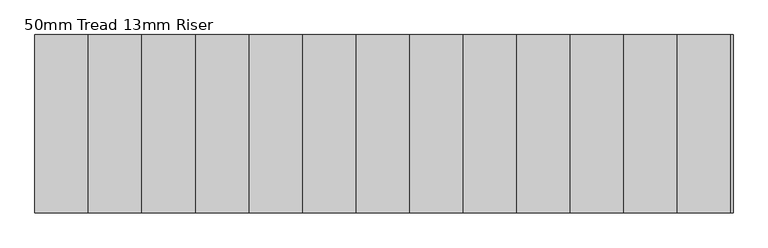
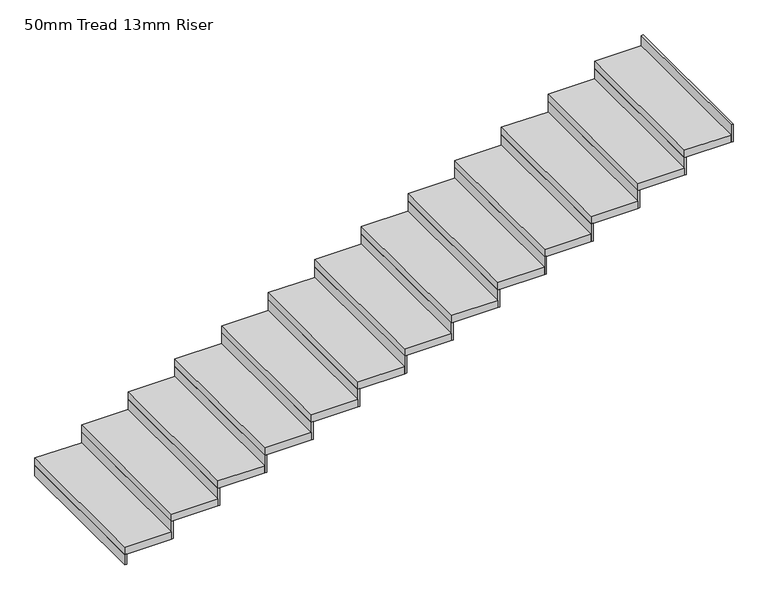
"""IFC4 building model written with IfcOpenShell, lengths in millimetres: stair flight geometry, 50mm Tread 13mm Riser."""

from ifc_helpers import new_model, si_unit, frame, origin, place, context, project, spatial, polyline, outline, extrude, source, transform, mapped, element, save


def stair_flight_50mm_tread_13mm_riser_be5964fb(model_context):
    return source(origin(), model_context, "Body", "SweptSolid", [
        extrude(outline(polyline([(17862.336337, -4574.4857187), (17849.836337, -4574.4857187), (17849.836337, -3574.4857187), (17862.336337, -3574.4857187), (17862.336337, -4574.4857187)])), frame((0.0, 0.0, 3000.0), z_axis=(0.0, 0.0, 1.0), x_axis=(1.0, 0.0, 0.0)), (0.0, 0.0, 1.0), 70.0),
        extrude(outline(polyline([(18149.836337, -3574.4857187), (18149.836337, -4574.4857187), (17849.836337, -4574.4857187), (17849.836337, -3574.4857187), (18149.836337, -3574.4857187)])), frame((0.0, 0.0, 3070.0), z_axis=(0.0, 0.0, 1.0), x_axis=(1.0, 0.0, 0.0)), (0.0, 0.0, 1.0), 50.0),
        extrude(outline(polyline([(18162.336337, -4574.4857187), (18149.836337, -4574.4857187), (18149.836337, -3574.4857187), (18162.336337, -3574.4857187), (18162.336337, -4574.4857187)])), frame((0.0, 0.0, 3070.0), z_axis=(0.0, 0.0, 1.0), x_axis=(1.0, 0.0, 0.0)), (0.0, 0.0, 1.0), 120.0),
        extrude(outline(polyline([(18449.836337, -3574.4857187), (18449.836337, -4574.4857187), (18149.836337, -4574.4857187), (18149.836337, -3574.4857187), (18449.836337, -3574.4857187)])), frame((0.0, 0.0, 3190.0), z_axis=(0.0, 0.0, 1.0), x_axis=(1.0, 0.0, 0.0)), (0.0, 0.0, 1.0), 50.0),
        extrude(outline(polyline([(18462.336337, -4574.4857187), (18449.836337, -4574.4857187), (18449.836337, -3574.4857187), (18462.336337, -3574.4857187), (18462.336337, -4574.4857187)])), frame((0.0, 0.0, 3190.0), z_axis=(0.0, 0.0, 1.0), x_axis=(1.0, 0.0, 0.0)), (0.0, 0.0, 1.0), 120.0),
        extrude(outline(polyline([(18749.836337, -3574.4857187), (18749.836337, -4574.4857187), (18449.836337, -4574.4857187), (18449.836337, -3574.4857187), (18749.836337, -3574.4857187)])), frame((0.0, 0.0, 3310.0), z_axis=(0.0, 0.0, 1.0), x_axis=(1.0, 0.0, 0.0)), (0.0, 0.0, 1.0), 50.0),
        extrude(outline(polyline([(18762.336337, -4574.4857187), (18749.836337, -4574.4857187), (18749.836337, -3574.4857187), (18762.336337, -3574.4857187), (18762.336337, -4574.4857187)])), frame((0.0, 0.0, 3310.0), z_axis=(0.0, 0.0, 1.0), x_axis=(1.0, 0.0, 0.0)), (0.0, 0.0, 1.0), 120.0),
        extrude(outline(polyline([(19049.836337, -3574.4857187), (19049.836337, -4574.4857187), (18749.836337, -4574.4857187), (18749.836337, -3574.4857187), (19049.836337, -3574.4857187)])), frame((0.0, 0.0, 3430.0), z_axis=(0.0, 0.0, 1.0), x_axis=(1.0, 0.0, 0.0)), (0.0, 0.0, 1.0), 50.0),
        extrude(outline(polyline([(19062.336337, -4574.4857187), (19049.836337, -4574.4857187), (19049.836337, -3574.4857187), (19062.336337, -3574.4857187), (19062.336337, -4574.4857187)])), frame((0.0, 0.0, 3430.0), z_axis=(0.0, 0.0, 1.0), x_axis=(1.0, 0.0, 0.0)), (0.0, 0.0, 1.0), 120.0),
        extrude(outline(polyline([(19349.836337, -3574.4857187), (19349.836337, -4574.4857187), (19049.836337, -4574.4857187), (19049.836337, -3574.4857187), (19349.836337, -3574.4857187)])), frame((0.0, 0.0, 3550.0), z_axis=(0.0, 0.0, 1.0), x_axis=(1.0, 0.0, 0.0)), (0.0, 0.0, 1.0), 50.0),
        extrude(outline(polyline([(19362.336337, -4574.4857187), (19349.836337, -4574.4857187), (19349.836337, -3574.4857187), (19362.336337, -3574.4857187), (19362.336337, -4574.4857187)])), frame((0.0, 0.0, 3550.0), z_axis=(0.0, 0.0, 1.0), x_axis=(1.0, 0.0, 0.0)), (0.0, 0.0, 1.0), 120.0),
        extrude(outline(polyline([(19649.836337, -3574.4857187), (19649.836337, -4574.4857187), (19349.836337, -4574.4857187), (19349.836337, -3574.4857187), (19649.836337, -3574.4857187)])), frame((0.0, 0.0, 3670.0), z_axis=(0.0, 0.0, 1.0), x_axis=(1.0, 0.0, 0.0)), (0.0, 0.0, 1.0), 50.0),
        extrude(outline(polyline([(19662.336337, -4574.4857187), (19649.836337, -4574.4857187), (19649.836337, -3574.4857187), (19662.336337, -3574.4857187), (19662.336337, -4574.4857187)])), frame((0.0, 0.0, 3670.0), z_axis=(0.0, 0.0, 1.0), x_axis=(1.0, 0.0, 0.0)), (0.0, 0.0, 1.0), 120.0),
        extrude(outline(polyline([(19949.836337, -3574.4857187), (19949.836337, -4574.4857187), (19649.836337, -4574.4857187), (19649.836337, -3574.4857187), (19949.836337, -3574.4857187)])), frame((0.0, 0.0, 3790.0), z_axis=(0.0, 0.0, 1.0), x_axis=(1.0, 0.0, 0.0)), (0.0, 0.0, 1.0), 50.0),
        extrude(outline(polyline([(19962.336337, -4574.4857187), (19949.836337, -4574.4857187), (19949.836337, -3574.4857187), (19962.336337, -3574.4857187), (19962.336337, -4574.4857187)])), frame((0.0, 0.0, 3790.0), z_axis=(0.0, 0.0, 1.0), x_axis=(1.0, 0.0, 0.0)), (0.0, 0.0, 1.0), 120.0),
        extrude(outline(polyline([(20249.836337, -3574.4857187), (20249.836337, -4574.4857187), (19949.836337, -4574.4857187), (19949.836337, -3574.4857187), (20249.836337, -3574.4857187)])), frame((0.0, 0.0, 3910.0), z_axis=(0.0, 0.0, 1.0), x_axis=(1.0, 0.0, 0.0)), (0.0, 0.0, 1.0), 50.0),
        extrude(outline(polyline([(20262.336337, -4574.4857187), (20249.836337, -4574.4857187), (20249.836337, -3574.4857187), (20262.336337, -3574.4857187), (20262.336337, -4574.4857187)])), frame((0.0, 0.0, 3910.0), z_axis=(0.0, 0.0, 1.0), x_axis=(1.0, 0.0, 0.0)), (0.0, 0.0, 1.0), 120.0),
        extrude(outline(polyline([(20549.836337, -3574.4857187), (20549.836337, -4574.4857187), (20249.836337, -4574.4857187), (20249.836337, -3574.4857187), (20549.836337, -3574.4857187)])), frame((0.0, 0.0, 4030.0), z_axis=(0.0, 0.0, 1.0), x_axis=(1.0, 0.0, 0.0)), (0.0, 0.0, 1.0), 50.0),
        extrude(outline(polyline([(20562.336337, -4574.4857187), (20549.836337, -4574.4857187), (20549.836337, -3574.4857187), (20562.336337, -3574.4857187), (20562.336337, -4574.4857187)])), frame((0.0, 0.0, 4030.0), z_axis=(0.0, 0.0, 1.0), x_axis=(1.0, 0.0, 0.0)), (0.0, 0.0, 1.0), 120.0),
        extrude(outline(polyline([(20849.836337, -3574.4857187), (20849.836337, -4574.4857187), (20549.836337, -4574.4857187), (20549.836337, -3574.4857187), (20849.836337, -3574.4857187)])), frame((0.0, 0.0, 4150.0), z_axis=(0.0, 0.0, 1.0), x_axis=(1.0, 0.0, 0.0)), (0.0, 0.0, 1.0), 50.0),
        extrude(outline(polyline([(20862.336337, -4574.4857187), (20849.836337, -4574.4857187), (20849.836337, -3574.4857187), (20862.336337, -3574.4857187), (20862.336337, -4574.4857187)])), frame((0.0, 0.0, 4150.0), z_axis=(0.0, 0.0, 1.0), x_axis=(1.0, 0.0, 0.0)), (0.0, 0.0, 1.0), 120.0),
        extrude(outline(polyline([(21149.836337, -3574.4857187), (21149.836337, -4574.4857187), (20849.836337, -4574.4857187), (20849.836337, -3574.4857187), (21149.836337, -3574.4857187)])), frame((0.0, 0.0, 4270.0), z_axis=(0.0, 0.0, 1.0), x_axis=(1.0, 0.0, 0.0)), (0.0, 0.0, 1.0), 50.0),
        extrude(outline(polyline([(21162.336337, -4574.4857187), (21149.836337, -4574.4857187), (21149.836337, -3574.4857187), (21162.336337, -3574.4857187), (21162.336337, -4574.4857187)])), frame((0.0, 0.0, 4270.0), z_axis=(0.0, 0.0, 1.0), x_axis=(1.0, 0.0, 0.0)), (0.0, 0.0, 1.0), 120.0),
        extrude(outline(polyline([(21449.836337, -3574.4857187), (21449.836337, -4574.4857187), (21149.836337, -4574.4857187), (21149.836337, -3574.4857187), (21449.836337, -3574.4857187)])), frame((0.0, 0.0, 4390.0), z_axis=(0.0, 0.0, 1.0), x_axis=(1.0, 0.0, 0.0)), (0.0, 0.0, 1.0), 50.0),
        extrude(outline(polyline([(21462.336337, -4574.4857187), (21449.836337, -4574.4857187), (21449.836337, -3574.4857187), (21462.336337, -3574.4857187), (21462.336337, -4574.4857187)])), frame((0.0, 0.0, 4390.0), z_axis=(0.0, 0.0, 1.0), x_axis=(1.0, 0.0, 0.0)), (0.0, 0.0, 1.0), 120.0),
        extrude(outline(polyline([(21762.336337, -4574.4857187), (21749.836337, -4574.4857187), (21749.836337, -3574.4857187), (21762.336337, -3574.4857187), (21762.336337, -4574.4857187)])), frame((0.0, 0.0, 4510.0), z_axis=(0.0, 0.0, 1.0), x_axis=(1.0, 0.0, 0.0)), (0.0, 0.0, 1.0), 120.0),
        extrude(outline(polyline([(21749.836337, -3574.4857187), (21749.836337, -4574.4857187), (21449.836337, -4574.4857187), (21449.836337, -3574.4857187), (21749.836337, -3574.4857187)])), frame((0.0, 0.0, 4510.0), z_axis=(0.0, 0.0, 1.0), x_axis=(1.0, 0.0, 0.0)), (0.0, 0.0, 1.0), 50.0),
    ])


if __name__ == "__main__":
    model = new_model("IFC4")
    model_context = context("Model", 3, world=origin())
    ifc_project = project(units=[si_unit("LENGTHUNIT", "METRE", prefix="MILLI")], contexts=[model_context])
    site = spatial("IfcSite", under=ifc_project)
    building = spatial("IfcBuilding", under=site)
    placement = place(None, origin())
    stair_flight_50mm_tread_13mm_riser_shape = stair_flight_50mm_tread_13mm_riser_be5964fb(model_context)
    element("IfcStairFlight", 1, ObjectType="50mm Tread 13mm Riser", at=placement, inside=building, context=model_context, shape_type="MappedRepresentation", body=[
        mapped(stair_flight_50mm_tread_13mm_riser_shape, transform((0.0, 0.0, 0.0), x_axis=(1.0, 0.0, 0.0), y_axis=(0.0, 1.0, 0.0), z_axis=(0.0, 0.0, 1.0))),
    ])
    save(model, "model.ifc")
